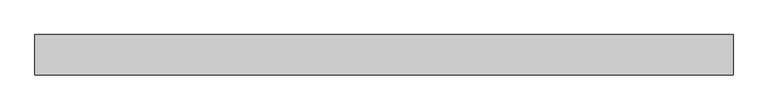
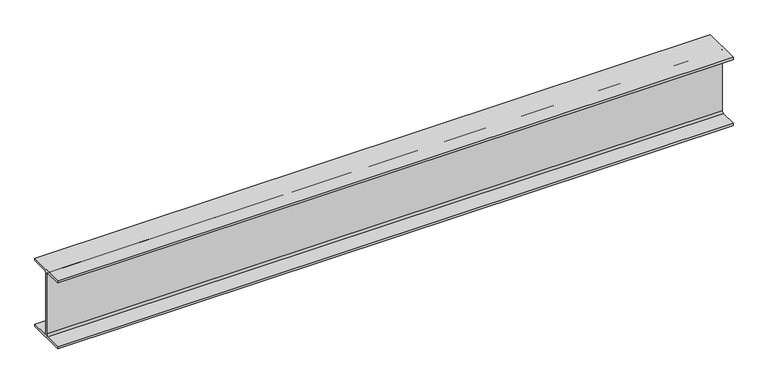
"""IFC4 building model written with IfcOpenShell, lengths in millimetres: beam geometry, Steel Beam_H-KSD3502 : H_SB_ASB_H-200x200x8x12."""

from ifc_helpers import new_model, si_unit, point, frame, frame_2d, origin, place, context, project, spatial, polyline, circle_curve, trimmed, segment, composite_curve, outline, extrude, source, transform, mapped, element, save


def beam_c1fe6c0d(model_context):
    return source(origin(), model_context, "Body", "SweptSolid", [
        extrude(outline(composite_curve([segment(polyline([(82.5, -141.5), (82.5, -151.7), (-82.5, -151.7), (-82.5, -141.5), (-11.9, -141.5)]), True, "CONTINUOUS"), segment(trimmed(circle_curve(frame_2d((-11.9, -132.6)), 8.9), [point((-11.9, -141.5))], [point((-3.0, -132.6))], True, "CARTESIAN"), True, "CONTINUOUS"), segment(polyline([(-3.0, -132.6), (-3.0, 132.6)]), True, "CONTINUOUS"), segment(trimmed(circle_curve(frame_2d((-11.9, 132.6)), 8.9), [point((-3.0, 132.6))], [point((-11.9, 141.5))], True, "CARTESIAN"), True, "CONTINUOUS"), segment(polyline([(-11.9, 141.5), (-82.5, 141.5), (-82.5, 151.7), (82.5, 151.7), (82.5, 141.5), (11.9, 141.5)]), True, "CONTINUOUS"), segment(trimmed(circle_curve(frame_2d((11.9, 132.6)), 8.9), [point((11.9, 141.5))], [point((3.0, 132.6))], True, "CARTESIAN"), True, "CONTINUOUS"), segment(polyline([(3.0, 132.6), (3.0, -132.6)]), True, "CONTINUOUS"), segment(trimmed(circle_curve(frame_2d((11.9, -132.6)), 8.9), [point((3.0, -132.6))], [point((11.9, -141.5))], True, "CARTESIAN"), True, "CONTINUOUS"), segment(polyline([(11.9, -141.5), (82.5, -141.5)]), True, "CONTINUOUS")], self_intersect=False)), frame((-1432.8225766, 0.0, 0.0), z_axis=(1.0, 0.0, 0.0), x_axis=(0.0, 1.0, 0.0)), (0.0, 0.0, 1.0), 2841.3927387),
    ])


if __name__ == "__main__":
    model = new_model("IFC4")
    model_context = context("Model", 3, world=origin())
    ifc_project = project(units=[si_unit("LENGTHUNIT", "METRE", prefix="MILLI")], contexts=[model_context])
    site = spatial("IfcSite", under=ifc_project)
    building = spatial("IfcBuilding", under=site)
    placement = place(None, origin())
    beam_shape = beam_c1fe6c0d(model_context)
    element("IfcBeam", 1, ObjectType="Steel Beam_H-KSD3502 : H_SB_ASB_H-200x200x8x12", at=placement, inside=building, context=model_context, shape_type="MappedRepresentation", body=[
        mapped(beam_shape, transform((0.0, 0.0, 0.0), x_axis=(1.0, 0.0, 0.0), y_axis=(0.0, 1.0, 0.0), z_axis=(0.0, 0.0, 1.0))),
    ])
    save(model, "model.ifc")

# Revit data of these elements
# Type "Steel Beam_H-KSD3502 : H_SB_ASB_H-200x200x8x12"
#   Width = 20.0 cm
#   Web Thickness = 0.8 cm
#   Web Fillet = 1.3 cm
#   Warping Constant = 141376.0 cm⁶
#   Torsional Moment of Inertia = 26.2485 cm⁴
#   Torsional Modulus = 1.0 cm³
#   Section Area = 63.53 cm²
#   Plastic Modulus weak axis = 244.0 cm³
#   Plastic Modulus strong axis = 525.0 cm³
#   Perimeter = 1.16 m²/m
#   Nominal Weight = 49.90 kgf/m
#   Moment of Inertia weak axis = 1600.00 cm⁴
#   Moment of Inertia strong axis = 4720.00 cm⁴
#   Height = 20.0 cm
#   Flange Thickness = 1.2 cm
#   Elastic Modulus weak axis = 160.0 cm³
#   Elastic Modulus strong axis = 472.0 cm³
#   Centroid Vertical = 10.0 cm
#   Centroid Horizontal = 10.0 cm
#   Length [instance default] = 1.5240 m
#   Structural Material [instance default] = Steel, 45-345
#   Assembly Code = ""
# Element 1 (IfcBeam, "Steel Beam_H-KSD3502 : H_SB_ASB_H-200x200x8x12")
#   Structural Material = none
# Materials
#   "Steel, 45-345": class "Metal", colour RGB 189 187 185, transparency 0, Description = "Steel 345 MPa", Cost = 0
